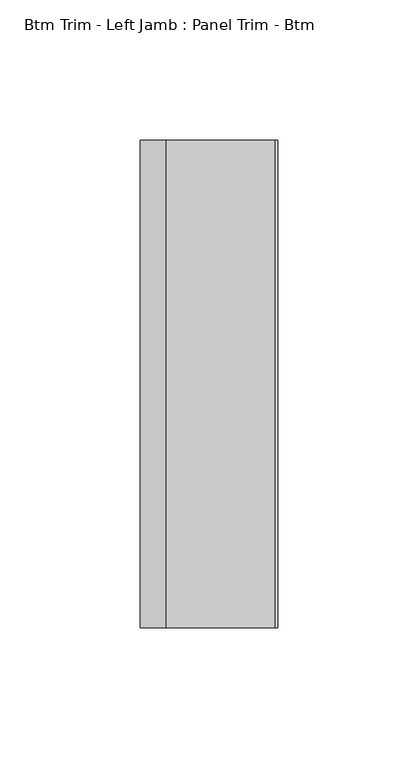
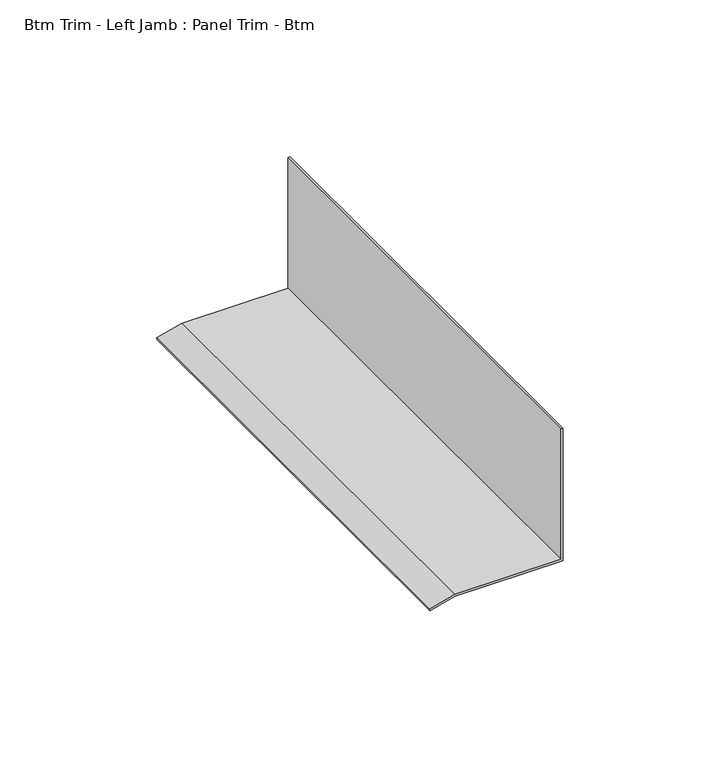
"""IFC4 building model written with IfcOpenShell, lengths in millimetres: proxy geometry, Btm Trim - Left Jamb : Panel Trim - Btm."""

from ifc_helpers import new_model, si_unit, frame, origin, place, context, project, spatial, polyline, outline, extrude, source, transform, mapped, element, save


def btm_trim_left_jamb_panel_trim_btm_7869e14d(model_context):
    return source(origin(), model_context, "Body", "SweptSolid", [
        extrude(outline(polyline([(12.7, 587326.9015748), (10.2077022, 587317.6001928), (9.4409986, 587317.8056304), (11.90625, 587327.0060739), (11.90625, 587366.6808739), (63.5, 587366.6808739), (63.5, 587365.8934739), (12.7, 587365.8934739), (12.7, 587326.9015748)])), frame((0.0, -531775.7413841, 0.0), z_axis=(0.0, 1.0, 0.0), x_axis=(0.0, 0.0, 1.0)), (0.0, 0.0, 1.0), 174.0154),
    ])


if __name__ == "__main__":
    model = new_model("IFC4")
    model_context = context("Model", 3, world=origin())
    ifc_project = project(units=[si_unit("LENGTHUNIT", "METRE", prefix="MILLI")], contexts=[model_context])
    site = spatial("IfcSite", under=ifc_project)
    building = spatial("IfcBuilding", under=site)
    placement = place(None, origin())
    btm_trim_left_jamb_panel_trim_btm_shape = btm_trim_left_jamb_panel_trim_btm_7869e14d(model_context)
    element("IfcBuildingElementProxy", 1, Name="Btm Trim - Left Jamb : Panel Trim - Btm", ObjectType="Btm Trim - Left Jamb : Panel Trim - Btm", at=placement, inside=building, context=model_context, shape_type="MappedRepresentation", body=[
        mapped(btm_trim_left_jamb_panel_trim_btm_shape, transform((0.0, 0.0, 0.0), x_axis=(1.0, 0.0, 0.0), y_axis=(0.0, 1.0, 0.0), z_axis=(0.0, 0.0, 1.0))),
    ])
    save(model, "model.ifc")

# Revit data of these elements
# Element 1 (IfcBuildingElementProxy, "Btm Trim - Left Jamb : Panel Trim - Btm")
#   Materials on its faces: "BASE TRIM BY MTL PANEL MFR."
# Materials
#   "BASE TRIM BY MTL PANEL MFR.": class "Generic", colour RGB 239 242 240, transparency 0, Cost = 0
